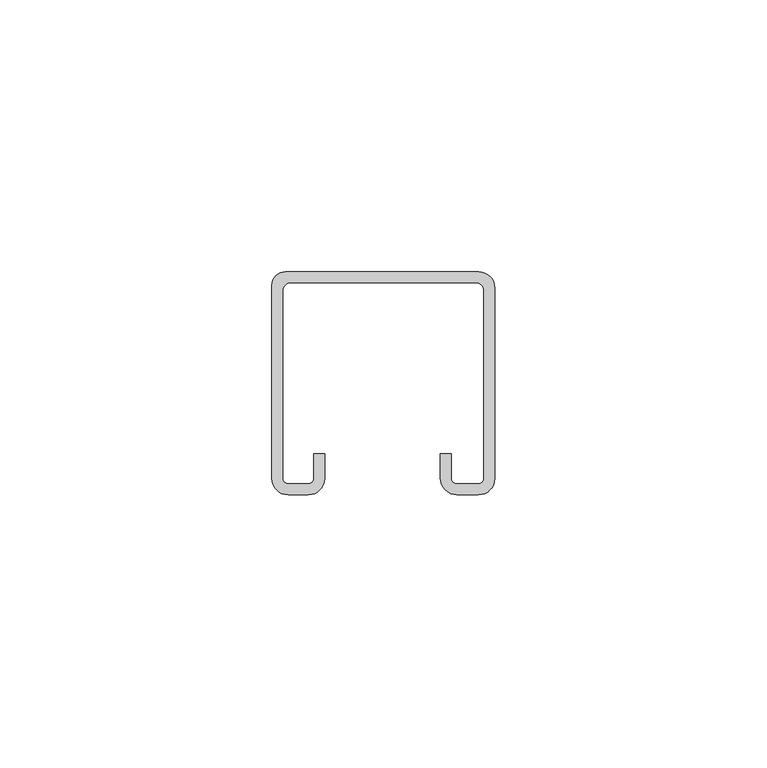
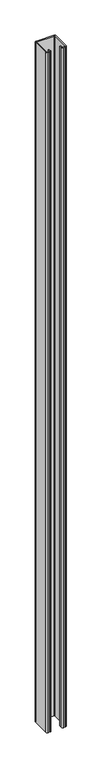
"""IFC4 building model written with IfcOpenShell, lengths in millimetres: proxy geometry, TN_Профиль монтажный : Профиль монтажный 41х41x2,0-3000."""

from ifc_helpers import new_model, si_unit, point, frame_2d, origin, origin_with_axes, place, context, project, spatial, polyline, circle_curve, trimmed, segment, composite_curve, outline, extrude, source, transform, mapped, element, save


def generic_models_234b3ffc(model_context):
    return source(origin(), model_context, "Body", "SweptSolid", [
        extrude(outline(composite_curve([segment(polyline([(20.7157599, -2.9315199), (20.7157599, -38.0)]), True, "CONTINUOUS"), segment(trimmed(circle_curve(frame_2d((17.7157599, -38.0)), 3.0), [point((20.7157599, -38.0))], [point((17.7157599, -41.0))], False, "CARTESIAN"), True, "CONTINUOUS"), segment(polyline([(17.7157599, -41.0), (13.7568638, -41.0)]), True, "CONTINUOUS"), segment(trimmed(circle_curve(frame_2d((13.7568638, -37.9588961)), 3.0411039), [point((13.7568638, -41.0))], [point((10.7157599, -37.9588961))], False, "CARTESIAN"), True, "CONTINUOUS"), segment(polyline([(10.7157599, -37.9588961), (10.7157599, -33.5), (12.7157599, -33.5), (12.7157599, -38.0)]), True, "CONTINUOUS"), segment(trimmed(circle_curve(frame_2d((13.7157599, -38.0)), 1.0), [point((12.7157599, -38.0))], [point((13.7157599, -39.0))], True, "CARTESIAN"), True, "CONTINUOUS"), segment(polyline([(13.7157599, -39.0), (17.7157599, -39.0)]), True, "CONTINUOUS"), segment(trimmed(circle_curve(frame_2d((17.7157599, -38.0)), 1.0), [point((17.7157599, -39.0))], [point((18.7157599, -38.0))], True, "CARTESIAN"), True, "CONTINUOUS"), segment(polyline([(18.7157599, -38.0), (18.7157599, -3.5)]), True, "CONTINUOUS"), segment(trimmed(circle_curve(frame_2d((17.2157599, -3.5)), 1.5), [point((18.7157599, -3.5))], [point((17.2157599, -2.0))], True, "CARTESIAN"), True, "CONTINUOUS"), segment(polyline([(17.2157599, -2.0), (-16.7842401, -2.0)]), True, "CONTINUOUS"), segment(trimmed(circle_curve(frame_2d((-16.7842401, -3.5)), 1.5), [point((-16.7842401, -2.0))], [point((-18.2842401, -3.5))], True, "CARTESIAN"), True, "CONTINUOUS"), segment(polyline([(-18.2842401, -3.5), (-18.2842401, -38.0)]), True, "CONTINUOUS"), segment(trimmed(circle_curve(frame_2d((-17.2842401, -38.0)), 1.0), [point((-18.2842401, -38.0))], [point((-17.2842401, -39.0))], True, "CARTESIAN"), True, "CONTINUOUS"), segment(polyline([(-17.2842401, -39.0), (-13.5684801, -39.0)]), True, "CONTINUOUS"), segment(trimmed(circle_curve(frame_2d((-13.5684801, -38.0)), 1.0), [point((-13.5684801, -39.0))], [point((-12.5684801, -38.0))], True, "CARTESIAN"), True, "CONTINUOUS"), segment(polyline([(-12.5684801, -38.0), (-12.5684801, -33.5), (-10.5684801, -33.5), (-10.5684801, -38.0)]), True, "CONTINUOUS"), segment(trimmed(circle_curve(frame_2d((-13.5684801, -38.0)), 3.0), [point((-10.5684801, -38.0))], [point((-13.5684801, -41.0))], False, "CARTESIAN"), True, "CONTINUOUS"), segment(polyline([(-13.5684801, -41.0), (-17.2842401, -41.0)]), True, "CONTINUOUS"), segment(trimmed(circle_curve(frame_2d((-17.2842401, -38.0)), 3.0), [point((-17.2842401, -41.0))], [point((-20.2842401, -38.0))], False, "CARTESIAN"), True, "CONTINUOUS"), segment(polyline([(-20.2842401, -38.0), (-20.2842401, -2.5)]), True, "CONTINUOUS"), segment(trimmed(circle_curve(frame_2d((-17.7842401, -2.5)), 2.5), [point((-20.2842401, -2.5))], [point((-17.7842401, 0.0))], False, "CARTESIAN"), True, "CONTINUOUS"), segment(polyline([(-17.7842401, 0.0), (17.7842401, 0.0)]), True, "CONTINUOUS"), segment(trimmed(circle_curve(frame_2d((17.7842401, -2.9315199)), 2.9315199), [point((17.7842401, 0.0))], [point((20.7157599, -2.9315199))], False, "CARTESIAN"), True, "CONTINUOUS")], self_intersect=False)), origin_with_axes(), (0.0, 0.0, 1.0), 1450.0),
    ])


if __name__ == "__main__":
    model = new_model("IFC4")
    model_context = context("Model", 3, world=origin())
    ifc_project = project(units=[si_unit("LENGTHUNIT", "METRE", prefix="MILLI")], contexts=[model_context])
    site = spatial("IfcSite", under=ifc_project)
    building = spatial("IfcBuilding", under=site)
    placement = place(None, origin())
    generic_models_shape = generic_models_234b3ffc(model_context)
    element("IfcBuildingElementProxy", 1, Name="TN_Профиль монтажный : Профиль монтажный 41х41x2,0-3000", ObjectType="TN_Профиль монтажный : Профиль монтажный 41х41x2,0-3000", at=placement, inside=building, context=model_context, shape_type="MappedRepresentation", body=[
        mapped(generic_models_shape, transform((0.0, 0.0, 0.0), x_axis=(1.0, 0.0, 0.0), y_axis=(0.0, 1.0, 0.0), z_axis=(0.0, 0.0, 1.0))),
    ])
    save(model, "model.ifc")

# Revit data of these elements
# Type "TN_Профиль монтажный : Профиль монтажный 41х41x2,0-3000"
#   Description = "Профиль монтажный – траверса С-образной формы предназначен для горизонтального и вертикального монтажа тяжелых инженерных систем, оборудования систем вентиляции и кондиционирования, установок электроснабжения, элементов трубопроводов, также для изготовления стенных консолей пристенного монтажа, рам оснований различного типа под оборудование. Возможно замещение на основе сконструированных модулей серийных опор ГОСТ для раскрепления технологических трубопроводов. Рекомендуется для применения в сухих, влажных помещениях и на открытом воздухе."
#   Manufacturer = "ТехноНИКОЛЬ"
#   Model = "Комплектующие к опорам"
#   URL = "https://nav.tn.ru/knowledge-base/polimernye-membrany/opory-pod-oborudovanie-na-ploskoy-krovle/?sphrase_id=266812"
#   ADSK_Обозначение = "ТехноНИКОЛЬ"
#   ADSK_Наименование краткое = "П41х41x2,0"
#   ADSK_Наименование = "Профиль монтажный 41х41x2,0-3000"
#   ADSK_Масса_Текст = ""
#   ADSK_Марка = "П41х41x2,0"
#   ADSK_Код изделия = "660816"
#   ADSK_Завод-изготовитель = "ТехноНИКОЛЬ"
#   ADSK_Единица измерения = "п.м."
#   ADSK_Группирование = "Комплектующие к опорам"
#   ADSK_URL страницы изделия = "https://nav.tn.ru/knowledge-base/polimernye-membrany/opory-pod-oborudovanie-na-ploskoy-krovle/?sphrase_id=266812"
#   ADSK_URL документации изделия = ""
#   Размер_Длина_Вводимая [instance default] = 1000 mm
#   ADSK_Размер_Длина [instance default] = 1000 mm
#   ADSK_Количество [instance default] = 1
#   Тип профиля = 1
#   Профиль монтажный 41х41x2,0 = yes
#   Профиль монтажный 41x62x2,5 = no
#   Профиль монтажный 41x124x2,5 = no
#   ADSK_Материал = TN_СтальГальванизированная_Серый
#   Default Elevation = 0
# Element 1 (IfcBuildingElementProxy, "TN_Профиль монтажный : Профиль монтажный 41х41x2,0-3000")
#   Размер_Длина_Вводимая = 1450 mm
#   ADSK_Размер_Длина = 1450 mm
#   ADSK_Количество = 1.45
#   Materials on its faces: "TN_СтальГальванизированная_Серый"
# Materials
#   "TN_СтальГальванизированная_Серый": class "Типовые", colour RGB 206 210 213, transparency 0, Cost = 0
